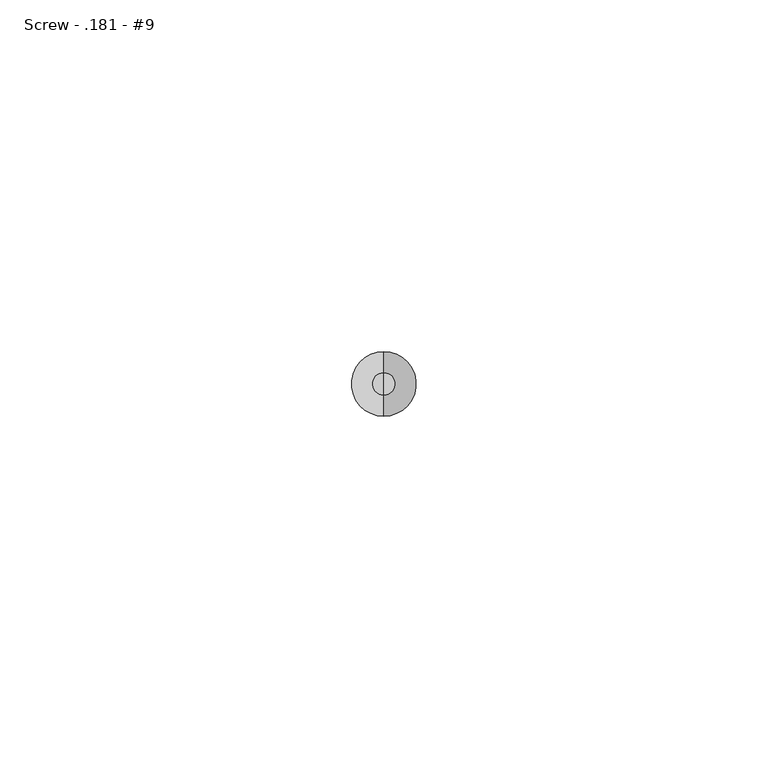
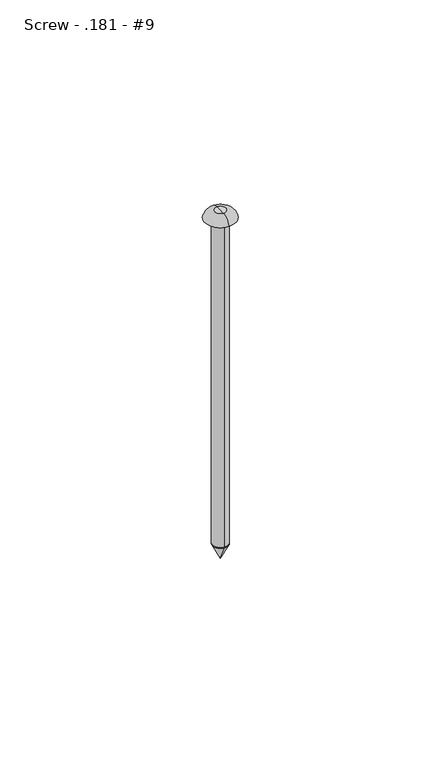
"""IFC4 building model written with IfcOpenShell, lengths in millimetres: fastener geometry, 060523 - W_P_C - Fastenings - Generic : Screw - .181 - #9."""

import ifcopenshell
import ifcopenshell.guid

model = None  # the IFC model being written
_history = None  # IfcOwnerHistory: only IFC2X3 demands one
_inside = {}  # id of a spatial element -> (the spatial element, [elements in it])
_under = {}  # id of a project, library or spatial element -> (it, [spatial elements below it])
_declared = {}  # id of a project -> (the project, [libraries it declares])
_typed = {}  # id of a type object -> (the type object, [elements of that type])
_made_of = {}  # id of a material, layer set ... -> (it, [elements and type objects made of it])


def new_model(schema):
    """Start an empty IFC model of exactly this schema.

    Asked for "IFC4X3", IfcOpenShell would pick the latest addendum, in which some entities
    have other attributes; the version numbers below select the first issue.
    IFC2X3 requires an IfcOwnerHistory on every rooted entity: one is made here for all.
    """
    global model, _history
    if schema == "IFC4X3":
        model = ifcopenshell.file(schema_version=(4, 3, 0, 0))
    else:
        model = ifcopenshell.file(schema=schema)
    _inside.clear()
    _under.clear()
    _declared.clear()
    _typed.clear()
    _made_of.clear()
    _history = None
    if model.schema == "IFC2X3":
        org = make("IfcOrganization", Name="unknown")
        user = make(
            "IfcPersonAndOrganization",
            ThePerson=make("IfcPerson", FamilyName="unknown"),
            TheOrganization=org,
        )
        app = make(
            "IfcApplication",
            ApplicationDeveloper=org,
            Version="unknown",
            ApplicationFullName="unknown",
            ApplicationIdentifier="unknown",
        )
        _history = make(
            "IfcOwnerHistory",
            OwningUser=user,
            OwningApplication=app,
            ChangeAction="ADDED",
            CreationDate=0,
        )
    return model


def make(cls, **values):
    """One entity of the class cls with the attributes given. An attribute that is None is left unset."""
    return model.create_entity(
        cls, **{name: value for name, value in values.items() if value is not None}
    )


def rooted(cls, **values):
    """An entity with a GlobalId (a new one), such as an element, a storey or a relation."""
    return make(cls, GlobalId=ifcopenshell.guid.new(), OwnerHistory=_history, **values)


def si_unit(unit_type, name, prefix=None):
    """IfcSIUnit, for example si_unit("LENGTHUNIT", "METRE", prefix="MILLI")."""
    return make("IfcSIUnit", UnitType=unit_type, Prefix=prefix, Name=name)


def assignment(units):
    """IfcUnitAssignment: the units of a project."""
    return None if units is None else make("IfcUnitAssignment", Units=units)


def point(xyz):
    """IfcCartesianPoint."""
    return None if xyz is None else make("IfcCartesianPoint", Coordinates=xyz)


def direction(xyz):
    """IfcDirection."""
    return None if xyz is None else make("IfcDirection", DirectionRatios=xyz)


def frame(location, z_axis=None, x_axis=None):
    """IfcAxis2Placement3D, a coordinate frame: its origin and axes. An axis left out is left unset."""
    return make(
        "IfcAxis2Placement3D",
        Location=point(location),
        Axis=direction(z_axis),
        RefDirection=direction(x_axis),
    )


def frame_2d(location, x_axis=None):
    """IfcAxis2Placement2D, a coordinate frame in the plane: its origin and x axis."""
    return make(
        "IfcAxis2Placement2D", Location=point(location), RefDirection=direction(x_axis)
    )


def origin():
    """The frame at (0, 0, 0) with its axes left unset."""
    return frame((0.0, 0.0, 0.0))


def origin_2d():
    """The frame at (0, 0) in the plane with its x axis left unset."""
    return frame_2d((0.0, 0.0))


def place(relative_to, where):
    """IfcLocalPlacement: puts the frame where relative to a parent placement (None: the world)."""
    return make(
        "IfcLocalPlacement", PlacementRelTo=relative_to, RelativePlacement=where
    )


def context(
    kind, dimensions, precision=None, world=None, true_north=None, identifier=None
):
    """IfcGeometricRepresentationContext, for example the 3D "Model" context."""
    return make(
        "IfcGeometricRepresentationContext",
        ContextIdentifier=identifier,
        ContextType=kind,
        CoordinateSpaceDimension=dimensions,
        Precision=precision,
        WorldCoordinateSystem=world,
        TrueNorth=true_north,
    )


def project(units=None, contexts=None):
    """IfcProject with its units and contexts."""
    return rooted(
        "IfcProject",
        Name="project",
        RepresentationContexts=contexts,
        UnitsInContext=assignment(units),
    )


def spatial(cls, under=None, at=None, **own):
    """A site, building, storey or space (cls), placed at a placement, below another one or the project."""
    s = rooted(cls, ObjectPlacement=at, **own)
    if under is not None:
        _under.setdefault(under.id(), (under, []))[1].append(s)
    return s


def polyline(points):
    """IfcPolyline through the points."""
    return make("IfcPolyline", Points=[point(p) for p in points])


def circle_curve(where, radius):
    """IfcCircle in the frame where."""
    return make("IfcCircle", Position=where, Radius=radius)


def ellipse_curve(where, semi_axis1, semi_axis2):
    """IfcEllipse in the frame where."""
    return make(
        "IfcEllipse", Position=where, SemiAxis1=semi_axis1, SemiAxis2=semi_axis2
    )


def trimmed(basis, trim1, trim2, sense, master):
    """IfcTrimmedCurve: the piece of a basis curve between two trims."""
    return make(
        "IfcTrimmedCurve",
        BasisCurve=basis,
        Trim1=trim1,
        Trim2=trim2,
        SenseAgreement=sense,
        MasterRepresentation=master,
    )


def segment(curve, same_sense, transition):
    """IfcCompositeCurveSegment."""
    return make(
        "IfcCompositeCurveSegment",
        Transition=transition,
        SameSense=same_sense,
        ParentCurve=curve,
    )


def composite_curve(segments, self_intersect=None):
    """IfcCompositeCurve: segments joined end to end."""
    return make("IfcCompositeCurve", Segments=segments, SelfIntersect=self_intersect)


def outline(outer, holes=None, kind="AREA"):
    """IfcArbitraryClosedProfileDef: a profile drawn as a closed curve; with holes, ...WithVoids."""
    if holes is None:
        return make("IfcArbitraryClosedProfileDef", ProfileType=kind, OuterCurve=outer)
    return make(
        "IfcArbitraryProfileDefWithVoids",
        ProfileType=kind,
        OuterCurve=outer,
        InnerCurves=holes,
    )


def extrude(swept, where, along, depth):
    """IfcExtrudedAreaSolid: the profile swept, set in the frame where, extruded along a direction by depth."""
    return make(
        "IfcExtrudedAreaSolid",
        SweptArea=swept,
        Position=where,
        ExtrudedDirection=direction(along),
        Depth=depth,
    )


def shape(context_of_items, identifier, shape_type, items):
    """IfcShapeRepresentation: the items that make up one representation, for example the "Body"."""
    return make(
        "IfcShapeRepresentation",
        ContextOfItems=context_of_items,
        RepresentationIdentifier=identifier,
        RepresentationType=shape_type,
        Items=items,
    )


def source(mapping_origin, context_of_items, identifier, shape_type, items):
    """IfcRepresentationMap: a shape defined once, which mapped items show again and again."""
    return make(
        "IfcRepresentationMap",
        MappingOrigin=mapping_origin,
        MappedRepresentation=shape(context_of_items, identifier, shape_type, items),
    )


def transform(
    local_origin,
    x_axis=None,
    y_axis=None,
    z_axis=None,
    scale=None,
    scale2=None,
    scale3=None,
    uniform=True,
):
    """IfcCartesianTransformationOperator3D, or its non-uniform kind. x_axis, y_axis, z_axis: its Axis1, 2, 3."""
    if uniform:
        return make(
            "IfcCartesianTransformationOperator3D",
            Axis1=direction(x_axis),
            Axis2=direction(y_axis),
            LocalOrigin=point(local_origin),
            Scale=scale,
            Axis3=direction(z_axis),
        )
    return make(
        "IfcCartesianTransformationOperator3DnonUniform",
        Axis1=direction(x_axis),
        Axis2=direction(y_axis),
        LocalOrigin=point(local_origin),
        Scale=scale,
        Axis3=direction(z_axis),
        Scale2=scale2,
        Scale3=scale3,
    )


def mapped(mapping_source, mapping_target):
    """IfcMappedItem: shows the shape of a source again, moved by a transform."""
    return make(
        "IfcMappedItem", MappingSource=mapping_source, MappingTarget=mapping_target
    )


def made_of(thing, what):
    """Note that an element or type object is made of a material, layer set ...; save() writes the relation."""
    if what is not None:
        _made_of.setdefault(what.id(), (what, []))[1].append(thing)
    return thing


def element(
    cls,
    number,
    at=None,
    inside=None,
    cuts=None,
    type_object=None,
    material=None,
    context=None,
    identifier="Body",
    shape_type=None,
    held_by="IfcProductDefinitionShape",
    body=None,
    shapes=None,
    **own,
):
    """One element of the class cls, such as IfcWall. Its Tag is "e" and its number.

    at: its placement. inside: the storey or other place that contains it. cuts: it is an
    opening in that element (IfcRelVoidsElement). A single representation is given by context,
    identifier, shape_type and body (its items); several are given by shapes. held_by: the class
    of the entity that holds the representations. save() writes the other relations.
    """
    e = rooted(cls, Tag="e%d" % number, ObjectPlacement=at, **own)
    if body is not None:
        shapes = [shape(context, identifier, shape_type, body)]
    if shapes is not None:
        e.Representation = make(held_by, Representations=shapes)
    if inside is not None:
        _inside.setdefault(inside.id(), (inside, []))[1].append(e)
    if cuts is not None:
        rooted(
            "IfcRelVoidsElement", RelatingBuildingElement=cuts, RelatedOpeningElement=e
        )
    if type_object is not None:
        _typed.setdefault(type_object.id(), (type_object, []))[1].append(e)
    return made_of(e, material)


def aggregate(whole, parts):
    """IfcRelAggregates: a whole, such as a stair, and the parts it consists of."""
    return rooted("IfcRelAggregates", RelatingObject=whole, RelatedObjects=parts)


def save(model, path):
    """Write the relations noted so far, then the file.

    IfcRelAggregates (storeys below a building ...), IfcRelContainedInSpatialStructure (elements
    in a storey), IfcRelDefinesByType, IfcRelAssociatesMaterial and IfcRelDeclares: one each for
    every whole, place, type object, material and project.
    """
    for whole, parts in _under.values():
        aggregate(whole, parts)
    for where, things in _inside.values():
        rooted(
            "IfcRelContainedInSpatialStructure",
            RelatedElements=things,
            RelatingStructure=where,
        )
    for kind, things in _typed.values():
        rooted("IfcRelDefinesByType", RelatedObjects=things, RelatingType=kind)
    for what, things in _made_of.values():
        rooted("IfcRelAssociatesMaterial", RelatedObjects=things, RelatingMaterial=what)
    for by, libraries in _declared.values():
        rooted("IfcRelDeclares", RelatingContext=by, RelatedDefinitions=libraries)
    model.write(path)


def plane_surface(at):
    """IfcPlane: the flat surface through the origin of the frame at, square to its z axis."""
    return make("IfcPlane", Position=at)


def revolved_surface(curve, axis_point, axis_direction):
    """IfcSurfaceOfRevolution: the curve turned about the line through axis_point along axis_direction."""
    return make(
        "IfcSurfaceOfRevolution",
        SweptCurve=make("IfcArbitraryOpenProfileDef", ProfileType="CURVE", Curve=curve),
        AxisPosition=make("IfcAxis1Placement", Location=point(axis_point), Axis=direction(axis_direction)),
    )


def advanced_brep(points, edges, surfaces, faces):
    """IfcAdvancedBrep: a solid bounded by faces that lie on surfaces and meet in shared edges.

    An edge is (start, end): straight between two places in points (the first is 0);
    or (start, end, curve); or (start, end, curve, False) where it runs against its curve.
    A face is (place in surfaces, loops), or (place, loops, False) where it looks against
    its surface's normal. A loop lists edges by number (the first is 1), with a minus sign
    where the edge is run from its end to its start. The first loop is the outer one.
    """
    corners = [point(p) for p in points]
    vertices = [make("IfcVertexPoint", VertexGeometry=c) for c in corners]
    made = []
    for start, end, *more in edges:
        made.append(
            make(
                "IfcEdgeCurve",
                EdgeStart=vertices[start],
                EdgeEnd=vertices[end],
                EdgeGeometry=more[0] if more else make("IfcPolyline", Points=[corners[start], corners[end]]),
                SameSense=more[1] if len(more) > 1 else True,
            )
        )
    hull = []
    for where, loops, *sense in faces:
        bounds = []
        for j, loop in enumerate(loops):
            ring = [make("IfcOrientedEdge", EdgeElement=made[abs(k) - 1], Orientation=k > 0) for k in loop]
            bounds.append(
                make(
                    "IfcFaceOuterBound" if j == 0 else "IfcFaceBound",
                    Bound=make("IfcEdgeLoop", EdgeList=ring),
                    Orientation=True,
                )
            )
        hull.append(make("IfcAdvancedFace", Bounds=bounds, FaceSurface=surfaces[where], SameSense=sense[0] if sense else True))
    return make("IfcAdvancedBrep", Outer=make("IfcClosedShell", CfsFaces=hull))


def screw_181_9_330bfe3c(model_context):
    return source(origin(), model_context, "Body", "SolidModel", [
        advanced_brep(
        [(0.0, -2.2987, -101.6), (0.0, 2.2987, -101.6), (0.0, 0.0, -101.6), (0.0, 0.0, -106.1974)],
        [
            (0, 1, circle_curve(frame((0.0, 0.0, -101.6), z_axis=(0.0, 0.0, 1.0), x_axis=(0.0, 1.0, 0.0)), 2.2987)),
            (1, 2),
            (2, 0),
            (1, 0, circle_curve(frame((0.0, 0.0, -101.6), z_axis=(0.0, 0.0, 1.0), x_axis=(0.0, 1.0, 0.0)), 2.2987)),
            (3, 1),
            (0, 3),
        ],
        [
            plane_surface(frame((0.0, 0.0, -101.6), z_axis=(0.0, 0.0, 1.0), x_axis=(0.0, 1.0, 0.0))),
            revolved_surface(polyline([(0.0, 2.2987, -101.6), (0.0, 0.0, -106.1974)]), (0.0, 0.0, -103.0840259), (0.0, 0.0, -1.0)),
        ],
        [
            (0, [[1, 2, 3]]),
            (0, [[4, -3, -2]]),
            (1, [[5, -1, 6]]),
            (1, [[-6, -4, -5]]),
        ],
    ),
        advanced_brep(
        [(0.0, 4.5974, 0.0), (0.0, -4.5974, 0.0), (0.0, 0.0, 0.0), (0.0, 0.0, 2.2987), (0.0, -1.5875, 2.2987), (0.0, 1.5875, 2.2987)],
        [
            (0, 1, circle_curve(frame((0.0, 0.0, 0.0), z_axis=(0.0, 0.0, -1.0), x_axis=(0.0, -1.0, 0.0)), 4.5974)),
            (1, 2),
            (2, 0),
            (1, 0, circle_curve(frame((0.0, 0.0, 0.0), z_axis=(0.0, 0.0, -1.0), x_axis=(0.0, -1.0, 0.0)), 4.5974)),
            (3, 4),
            (4, 5, circle_curve(frame((0.0, 0.0, 2.2987), z_axis=(0.0, 0.0, 1.0), x_axis=(0.0, -1.0, 0.0)), 1.5875)),
            (5, 3),
            (5, 4, circle_curve(frame((0.0, 0.0, 2.2987), z_axis=(0.0, 0.0, 1.0), x_axis=(0.0, -1.0, 0.0)), 1.5875)),
            (4, 1, circle_curve(frame((0.0, -1.5875, -0.8212199), z_axis=(1.0, 0.0, 0.0), x_axis=(0.0, -1.0, 0.0)), 3.1199199)),
            (0, 5, circle_curve(frame((0.0, 1.5875, -0.8212199), z_axis=(1.0, 0.0, 0.0), x_axis=(0.0, 1.0, 0.0)), 3.1199199)),
        ],
        [
            plane_surface(frame((0.0, 0.0, 0.0), z_axis=(0.0, 0.0, -1.0), x_axis=(0.0, -1.0, 0.0))),
            plane_surface(frame((0.0, 0.0, 2.2987), z_axis=(0.0, 0.0, 1.0), x_axis=(0.0, -1.0, 0.0))),
            revolved_surface(trimmed(ellipse_curve(frame((0.0, -1.5875, -0.8212199), z_axis=(-1.0, 0.0, 0.0), x_axis=(0.0, -1.0, 0.0)), 3.1199199, 3.1199199), [point((0.0, -4.5974, 0.0))], [point((0.0, -1.5875, 2.2987))], True, "CARTESIAN"), (0.0, 0.0, 1.4840259), (0.0, 0.0, 1.0)),
        ],
        [
            (0, [[1, 2, 3]]),
            (0, [[4, -3, -2]]),
            (1, [[5, 6, 7]]),
            (1, [[-7, 8, -5]]),
            (2, [[-6, 9, -1, 10]]),
            (2, [[-8, -10, -4, -9]]),
        ],
    ),
        extrude(outline(composite_curve([segment(trimmed(circle_curve(origin_2d(), 2.2987), [point((0.0, -2.2987))], [point((0.0, 2.2987))], False, "CARTESIAN"), True, "CONTINUOUS"), segment(trimmed(circle_curve(origin_2d(), 2.2987), [point((0.0, 2.2987))], [point((0.0, -2.2987))], False, "CARTESIAN"), True, "CONTINUOUS")], self_intersect=False)), frame((0.0, 0.0, -101.6), z_axis=(0.0, 0.0, 1.0), x_axis=(1.0, 0.0, 0.0)), (0.0, 0.0, 1.0), 101.6),
    ])


if __name__ == "__main__":
    model = new_model("IFC4")
    model_context = context("Model", 3, world=origin())
    ifc_project = project(units=[si_unit("LENGTHUNIT", "METRE", prefix="MILLI")], contexts=[model_context])
    site = spatial("IfcSite", under=ifc_project)
    building = spatial("IfcBuilding", under=site)
    placement = place(None, origin())
    screw_181_9_shape = screw_181_9_330bfe3c(model_context)
    element("IfcFastener", 1, ObjectType="060523 - W_P_C - Fastenings - Generic : Screw - .181 - #9", at=placement, inside=building, context=model_context, shape_type="MappedRepresentation", body=[
        mapped(screw_181_9_shape, transform((0.0, 0.0, 0.0), x_axis=(1.0, 0.0, 0.0), y_axis=(0.0, 1.0, 0.0), z_axis=(0.0, 0.0, 1.0))),
    ])
    save(model, "model.ifc")

# Revit data of these elements
# Type "060523 - W_P_C - Fastenings - Generic : Screw - .181 - #9"
#   Washer_Thickness = 0' - 0.00333"
#   Washer Radius = 0' - 0.1005"
#   Washer Offset - Head = 0' - 0"
#   Washer Offset = 0' - 0"
#   Thickness_of_Substrate [instance default] = 0' - 1"
#   Side = 0' - 0 37/64"
#   Radius = 0' - 0.0905"
#   Length [instance default] = 0' - 4"
#   Head Size = 0' - 1"
#   Head Radius = 0' - 0 1/2"
#   Head Height = 0' - 0.01"
#   Double Diameter = 0' - 0.362"
#   Diameter = 0' - 0.181"
#   Default Elevation = 4' - 0"
#   Washer_Nut_Visibility = no
#   Washer_Head_Visibility = no
#   Round_Head_Visibility = yes
#   Point Visibility = yes
#   Nut_Visibility = no
#   Hex_Head_Visiblilty = no
#   Washer Material = none
#   Bolt Material (Size) = AT SILL - FASTENER AT 24" O.C.
# Element 1 (IfcFastener, "060523 - W_P_C - Fastenings - Generic : Screw - .181 - #9")
#   Materials on its faces: "AT SILL - FASTENER AT 24\" O.C."
# Materials
#   "AT SILL - FASTENER AT 24\" O.C.": class "Generic", colour RGB 120 120 120, transparency 0, Cost = 0
